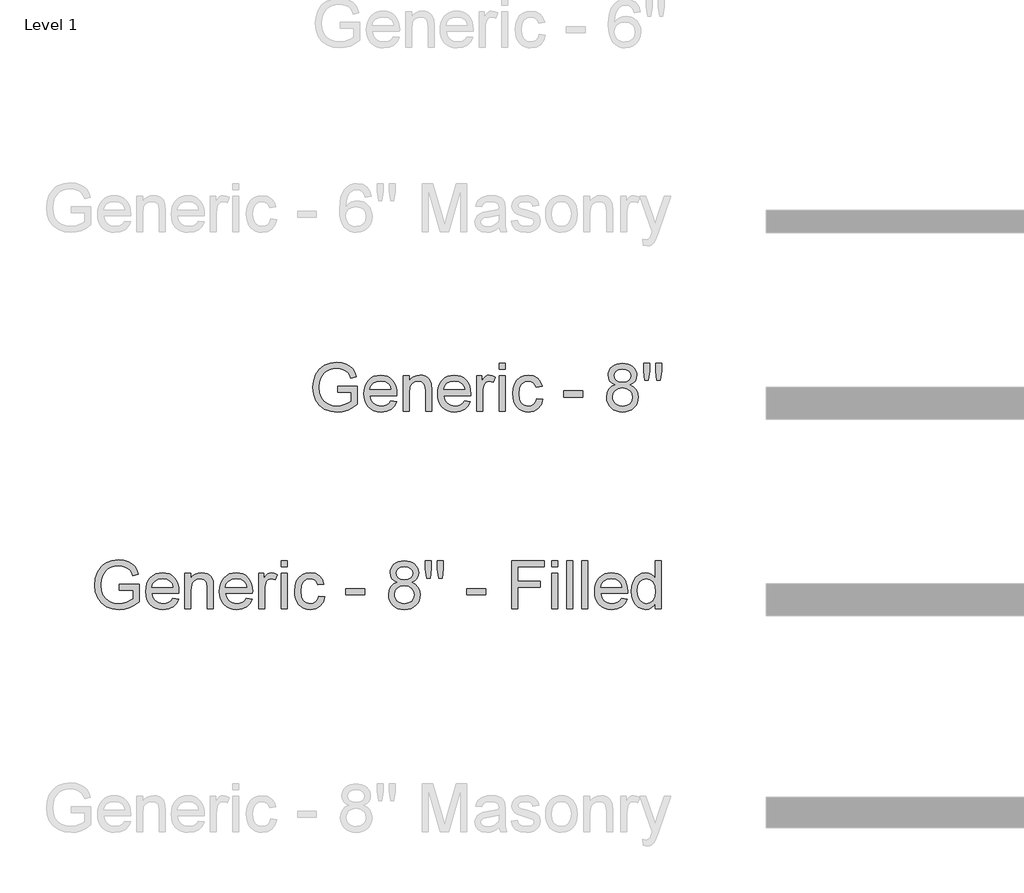
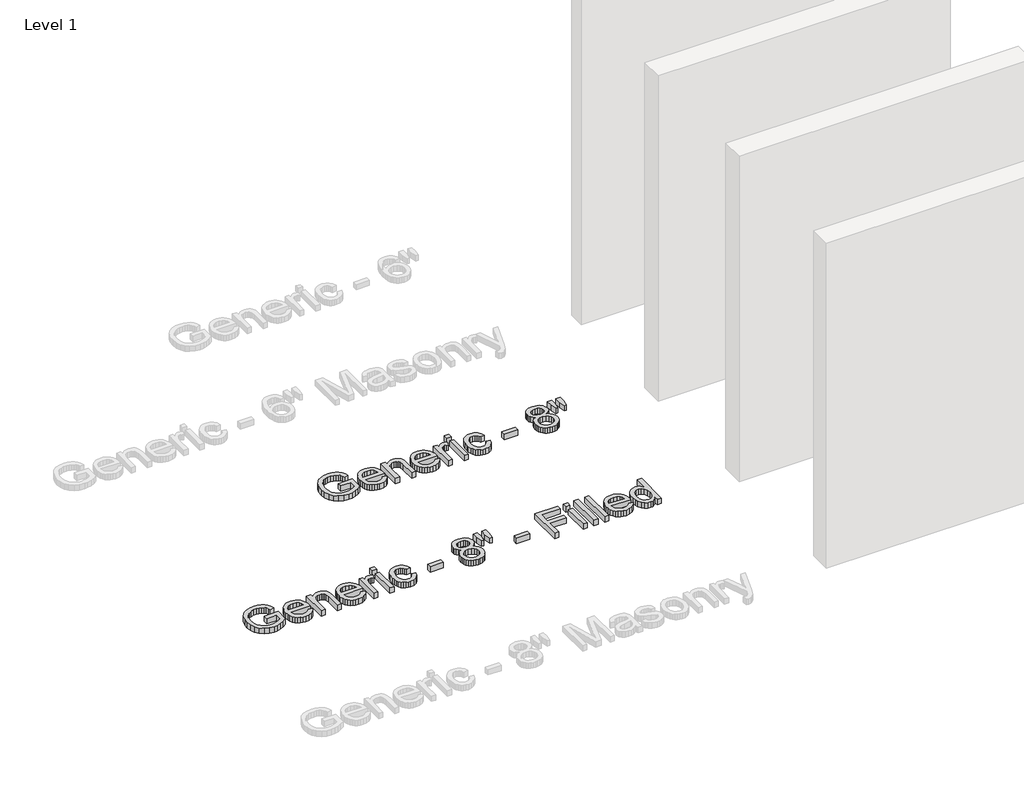
# One storey, part 23 of 42: 2 proxies.
"""IFC4 building model written with IfcOpenShell, lengths in millimetres."""

import ifcopenshell
import ifcopenshell.guid

model = None  # the IFC model being written
_history = None  # IfcOwnerHistory: only IFC2X3 demands one
_inside = {}  # id of a spatial element -> (the spatial element, [elements in it])
_under = {}  # id of a project, library or spatial element -> (it, [spatial elements below it])
_declared = {}  # id of a project -> (the project, [libraries it declares])
_typed = {}  # id of a type object -> (the type object, [elements of that type])
_made_of = {}  # id of a material, layer set ... -> (it, [elements and type objects made of it])


def new_model(schema):
    """Start an empty IFC model of exactly this schema.

    Asked for "IFC4X3", IfcOpenShell would pick the latest addendum, in which some entities
    have other attributes; the version numbers below select the first issue.
    IFC2X3 requires an IfcOwnerHistory on every rooted entity: one is made here for all.
    """
    global model, _history
    if schema == "IFC4X3":
        model = ifcopenshell.file(schema_version=(4, 3, 0, 0))
    else:
        model = ifcopenshell.file(schema=schema)
    _inside.clear()
    _under.clear()
    _declared.clear()
    _typed.clear()
    _made_of.clear()
    _history = None
    if model.schema == "IFC2X3":
        org = make("IfcOrganization", Name="unknown")
        user = make(
            "IfcPersonAndOrganization",
            ThePerson=make("IfcPerson", FamilyName="unknown"),
            TheOrganization=org,
        )
        app = make(
            "IfcApplication",
            ApplicationDeveloper=org,
            Version="unknown",
            ApplicationFullName="unknown",
            ApplicationIdentifier="unknown",
        )
        _history = make(
            "IfcOwnerHistory",
            OwningUser=user,
            OwningApplication=app,
            ChangeAction="ADDED",
            CreationDate=0,
        )
    return model


def make(cls, **values):
    """One entity of the class cls with the attributes given. An attribute that is None is left unset."""
    return model.create_entity(
        cls, **{name: value for name, value in values.items() if value is not None}
    )


def rooted(cls, **values):
    """An entity with a GlobalId (a new one), such as an element, a storey or a relation."""
    return make(cls, GlobalId=ifcopenshell.guid.new(), OwnerHistory=_history, **values)


def si_unit(unit_type, name, prefix=None):
    """IfcSIUnit, for example si_unit("LENGTHUNIT", "METRE", prefix="MILLI")."""
    return make("IfcSIUnit", UnitType=unit_type, Prefix=prefix, Name=name)


def assignment(units):
    """IfcUnitAssignment: the units of a project."""
    return None if units is None else make("IfcUnitAssignment", Units=units)


def point(xyz):
    """IfcCartesianPoint."""
    return None if xyz is None else make("IfcCartesianPoint", Coordinates=xyz)


def direction(xyz):
    """IfcDirection."""
    return None if xyz is None else make("IfcDirection", DirectionRatios=xyz)


def frame(location, z_axis=None, x_axis=None):
    """IfcAxis2Placement3D, a coordinate frame: its origin and axes. An axis left out is left unset."""
    return make(
        "IfcAxis2Placement3D",
        Location=point(location),
        Axis=direction(z_axis),
        RefDirection=direction(x_axis),
    )


def origin():
    """The frame at (0, 0, 0) with its axes left unset."""
    return frame((0.0, 0.0, 0.0))


def origin_with_axes():
    """The frame at (0, 0, 0) with the z axis (0, 0, 1) and the x axis (1, 0, 0) written out."""
    return frame((0.0, 0.0, 0.0), z_axis=(0.0, 0.0, 1.0), x_axis=(1.0, 0.0, 0.0))


def place(relative_to, where):
    """IfcLocalPlacement: puts the frame where relative to a parent placement (None: the world)."""
    return make(
        "IfcLocalPlacement", PlacementRelTo=relative_to, RelativePlacement=where
    )


def context(
    kind, dimensions, precision=None, world=None, true_north=None, identifier=None
):
    """IfcGeometricRepresentationContext, for example the 3D "Model" context."""
    return make(
        "IfcGeometricRepresentationContext",
        ContextIdentifier=identifier,
        ContextType=kind,
        CoordinateSpaceDimension=dimensions,
        Precision=precision,
        WorldCoordinateSystem=world,
        TrueNorth=true_north,
    )


def project(units=None, contexts=None):
    """IfcProject with its units and contexts."""
    return rooted(
        "IfcProject",
        Name="project",
        RepresentationContexts=contexts,
        UnitsInContext=assignment(units),
    )


def spatial(cls, under=None, at=None, **own):
    """A site, building, storey or space (cls), placed at a placement, below another one or the project."""
    s = rooted(cls, ObjectPlacement=at, **own)
    if under is not None:
        _under.setdefault(under.id(), (under, []))[1].append(s)
    return s


def polyline(points):
    """IfcPolyline through the points."""
    return make("IfcPolyline", Points=[point(p) for p in points])


def outline(outer, holes=None, kind="AREA"):
    """IfcArbitraryClosedProfileDef: a profile drawn as a closed curve; with holes, ...WithVoids."""
    if holes is None:
        return make("IfcArbitraryClosedProfileDef", ProfileType=kind, OuterCurve=outer)
    return make(
        "IfcArbitraryProfileDefWithVoids",
        ProfileType=kind,
        OuterCurve=outer,
        InnerCurves=holes,
    )


def extrude(swept, where, along, depth):
    """IfcExtrudedAreaSolid: the profile swept, set in the frame where, extruded along a direction by depth."""
    return make(
        "IfcExtrudedAreaSolid",
        SweptArea=swept,
        Position=where,
        ExtrudedDirection=direction(along),
        Depth=depth,
    )


def shape(context_of_items, identifier, shape_type, items):
    """IfcShapeRepresentation: the items that make up one representation, for example the "Body"."""
    return make(
        "IfcShapeRepresentation",
        ContextOfItems=context_of_items,
        RepresentationIdentifier=identifier,
        RepresentationType=shape_type,
        Items=items,
    )


def made_of(thing, what):
    """Note that an element or type object is made of a material, layer set ...; save() writes the relation."""
    if what is not None:
        _made_of.setdefault(what.id(), (what, []))[1].append(thing)
    return thing


def element(
    cls,
    number,
    at=None,
    inside=None,
    cuts=None,
    type_object=None,
    material=None,
    context=None,
    identifier="Body",
    shape_type=None,
    held_by="IfcProductDefinitionShape",
    body=None,
    shapes=None,
    **own,
):
    """One element of the class cls, such as IfcWall. Its Tag is "e" and its number.

    at: its placement. inside: the storey or other place that contains it. cuts: it is an
    opening in that element (IfcRelVoidsElement). A single representation is given by context,
    identifier, shape_type and body (its items); several are given by shapes. held_by: the class
    of the entity that holds the representations. save() writes the other relations.
    """
    e = rooted(cls, Tag="e%d" % number, ObjectPlacement=at, **own)
    if body is not None:
        shapes = [shape(context, identifier, shape_type, body)]
    if shapes is not None:
        e.Representation = make(held_by, Representations=shapes)
    if inside is not None:
        _inside.setdefault(inside.id(), (inside, []))[1].append(e)
    if cuts is not None:
        rooted(
            "IfcRelVoidsElement", RelatingBuildingElement=cuts, RelatedOpeningElement=e
        )
    if type_object is not None:
        _typed.setdefault(type_object.id(), (type_object, []))[1].append(e)
    return made_of(e, material)


def aggregate(whole, parts):
    """IfcRelAggregates: a whole, such as a stair, and the parts it consists of."""
    return rooted("IfcRelAggregates", RelatingObject=whole, RelatedObjects=parts)


def save(model, path):
    """Write the relations noted so far, then the file.

    IfcRelAggregates (storeys below a building ...), IfcRelContainedInSpatialStructure (elements
    in a storey), IfcRelDefinesByType, IfcRelAssociatesMaterial and IfcRelDeclares: one each for
    every whole, place, type object, material and project.
    """
    for whole, parts in _under.values():
        aggregate(whole, parts)
    for where, things in _inside.values():
        rooted(
            "IfcRelContainedInSpatialStructure",
            RelatedElements=things,
            RelatingStructure=where,
        )
    for kind, things in _typed.values():
        rooted("IfcRelDefinesByType", RelatedObjects=things, RelatingType=kind)
    for what, things in _made_of.values():
        rooted("IfcRelAssociatesMaterial", RelatedObjects=things, RelatingMaterial=what)
    for by, libraries in _declared.values():
        rooted("IfcRelDeclares", RelatingContext=by, RelatedDefinitions=libraries)
    model.write(path)


model = new_model("IFC4")

# Units and contexts
model_context = context("Model", 3, world=origin())
ifc_project = project(units=[si_unit("LENGTHUNIT", "METRE", prefix="MILLI")], contexts=[model_context])

# Site, building, storey
site = spatial("IfcSite", under=ifc_project)
building = spatial("IfcBuilding", under=site)
storey = spatial("IfcBuildingStorey", under=building, Name="Level 1", Elevation=0.0)

# Proxies
placement = place(None, origin())
element("IfcBuildingElementProxy", 1, Name="8\" Arial", ObjectType="8\" Arial", at=placement, inside=storey, context=model_context, shape_type="SweptSolid", body=[
    extrude(outline(polyline([(-15234.2304612, 12301.3438575), (-15234.2304612, 12339.4147443), (-15110.5000792, 12339.4147443), (-15110.5000792, 12225.57387), (-15140.5682722, 12204.6609073), (-15171.5845196, 12189.6593421), (-15203.474464, 12180.6249422), (-15236.1637484, 12177.6134755), (-15278.8726656, 12182.4002203), (-15317.4733474, 12196.7604547), (-15349.5398902, 12220.1922676), (-15372.6463903, 12252.1937479), (-15386.6162494, 12290.5806527), (-15391.2728691, 12333.1687394), (-15386.6348387, 12376.0635496), (-15372.7207475, 12415.9654824), (-15350.1068638, 12449.4355174), (-15335.7536004, 12462.4689404), (-15319.369456, 12473.0346339), (-15281.9306054, 12487.032377), (-15239.2123936, 12491.6982913), (-15207.8522442, 12488.9935481), (-15179.6522759, 12480.8793186), (-15155.9044449, 12467.9411657), (-15137.9007077, 12450.7646523), (-15124.5814741, 12428.5225547), (-15114.8871541, 12400.3876488), (-15149.9837528, 12390.4981412), (-15157.8191428, 12410.5652907), (-15167.3461592, 12425.7062757), (-15179.9497047, 12437.120106), (-15197.0146822, 12446.0057915), (-15217.3606713, 12451.7220013), (-15239.8072512, 12453.6274045), (-15266.083227, 12451.5732869), (-15288.5483963, 12445.4109339), (-15307.1191072, 12435.9118015), (-15321.7117078, 12423.8473457), (-15341.3048302, 12394.51343), (-15350.2276943, 12365.7743719), (-15353.2019823, 12334.7302406), (-15349.623542, 12298.3230962), (-15338.8882212, 12268.366439), (-15321.3213325, 12245.0740459), (-15297.2481888, 12228.6596938), (-15269.0761044, 12218.9281952), (-15239.2123936, 12215.6843623), (-15212.8434713, 12218.1288553), (-15187.1251745, 12225.4623342), (-15164.7901304, 12235.5656188), (-15148.570966, 12246.319529), (-15148.570966, 12301.3438575), (-15234.2304612, 12301.3438575)])), origin_with_axes(), (0.0, 0.0, 1.0), 50.8),
    extrude(outline(polyline([(-14896.7974844, 12248.9963882), (-14859.4701697, 12244.2375274), (-14872.9195283, 12216.1119162), (-14894.3808754, 12195.0874177), (-14923.370889, 12181.9819611), (-14959.4062474, 12177.6134755), (-14983.0286006, 12179.4979659), (-15004.0763357, 12185.1514368), (-15022.5494528, 12194.5738883), (-15038.4479517, 12207.7653204), (-15051.2327429, 12224.3585945), (-15060.3647366, 12243.9865718), (-15065.8439329, 12266.6492524), (-15067.6703316, 12292.3466362), (-15065.8253436, 12318.9153935), (-15060.2903794, 12342.3332644), (-15051.0654392, 12362.6002489), (-15038.1505229, 12379.7163471), (-15022.2938499, 12393.3144201), (-15004.2436394, 12403.0273295), (-14983.9998915, 12408.8550751), (-14961.5626062, 12410.7976569), (-14939.8479799, 12408.8597224), (-14920.210708, 12403.0459188), (-14902.6507903, 12393.3562461), (-14887.1682269, 12379.7907043), (-14874.5298265, 12362.7117847), (-14865.5023976, 12342.4819788), (-14860.0859402, 12319.1012865), (-14858.2804544, 12292.5697078), (-14858.503526, 12282.3084141), (-15029.5994449, 12282.3084141), (-15023.0095379, 12253.811017), (-15007.7012492, 12232.8608757), (-14985.607866, 12219.9784906), (-14958.6626754, 12215.6843623), (-14938.4003382, 12217.6734174), (-14921.3353606, 12223.6405828), (-14907.4677427, 12233.9576444), (-14896.7974844, 12248.9963882)]), holes=[polyline([(-15029.5994449, 12320.3793009), (-14896.3513412, 12320.3793009), (-14901.5005773, 12340.4929237), (-14911.5945673, 12354.881042), (-14933.7901918, 12368.2653381), (-14961.7113206, 12372.7267702), (-14987.3738495, 12369.1669192), (-15008.5935357, 12358.4873663), (-15023.3441453, 12341.8406479), (-15029.5994449, 12320.3793009)])]), origin_with_axes(), (0.0, 0.0, 1.0), 50.8),
    extrude(outline(polyline([(-14820.2095677, 12182.3723364), (-14820.2095677, 12406.0387961), (-14782.1386809, 12406.0387961), (-14782.1386809, 12374.8087718), (-14768.9123938, 12390.5539091), (-14753.0278368, 12401.8004357), (-14734.4850099, 12408.5483516), (-14713.2839131, 12410.7976569), (-14694.5180145, 12408.9852002), (-14677.3322065, 12403.5478299), (-14662.9998561, 12395.1640555), (-14652.7943303, 12384.5123865), (-14641.3805, 12356.5169004), (-14639.3728556, 12319.7100861), (-14639.3728556, 12182.3723364), (-14677.4437423, 12182.3723364), (-14677.4437423, 12314.5794392), (-14681.8308172, 12348.2632512), (-14687.9002237, 12358.2921786), (-14697.3342935, 12366.0718007), (-14709.4266333, 12371.0630278), (-14723.4708496, 12372.7267702), (-14745.7687151, 12368.9903209), (-14764.7762746, 12357.7809728), (-14772.3723273, 12348.6303898), (-14777.7980793, 12336.1244381), (-14782.1386809, 12301.0464287), (-14782.1386809, 12182.3723364), (-14820.2095677, 12182.3723364)])), origin_with_axes(), (0.0, 0.0, 1.0), 50.8),
    extrude(outline(polyline([(-14430.4291216, 12248.9963882), (-14393.1018069, 12244.2375274), (-14406.5511655, 12216.1119162), (-14428.0125126, 12195.0874177), (-14457.0025262, 12181.9819611), (-14493.0378846, 12177.6134755), (-14516.6602378, 12179.4979659), (-14537.7079729, 12185.1514368), (-14556.18109, 12194.5738883), (-14572.0795889, 12207.7653204), (-14584.8643801, 12224.3585945), (-14593.9963739, 12243.9865718), (-14599.4755701, 12266.6492524), (-14601.3019688, 12292.3466362), (-14599.4569808, 12318.9153935), (-14593.9220167, 12342.3332644), (-14584.6970764, 12362.6002489), (-14571.7821601, 12379.7163471), (-14555.9254871, 12393.3144201), (-14537.8752766, 12403.0273295), (-14517.6315287, 12408.8550751), (-14495.1942434, 12410.7976569), (-14473.4796172, 12408.8597224), (-14453.8423452, 12403.0459188), (-14436.2824275, 12393.3562461), (-14420.7998641, 12379.7907043), (-14408.1614637, 12362.7117847), (-14399.1340348, 12342.4819788), (-14393.7175774, 12319.1012865), (-14391.9120916, 12292.5697078), (-14392.1351632, 12282.3084141), (-14563.2310821, 12282.3084141), (-14556.6411751, 12253.811017), (-14541.3328865, 12232.8608757), (-14519.2395032, 12219.9784906), (-14492.2943126, 12215.6843623), (-14472.0319754, 12217.6734174), (-14454.9669978, 12223.6405828), (-14441.0993799, 12233.9576444), (-14430.4291216, 12248.9963882)]), holes=[polyline([(-14563.2310821, 12320.3793009), (-14429.9829784, 12320.3793009), (-14435.1322146, 12340.4929237), (-14445.2262045, 12354.881042), (-14467.421829, 12368.2653381), (-14495.3429578, 12372.7267702), (-14521.0054867, 12369.1669192), (-14542.2251729, 12358.4873663), (-14556.9757826, 12341.8406479), (-14563.2310821, 12320.3793009)])]), origin_with_axes(), (0.0, 0.0, 1.0), 50.8),
    extrude(outline(polyline([(-14353.8412049, 12182.3723364), (-14353.8412049, 12406.0387961), (-14320.529179, 12406.0387961), (-14320.529179, 12372.9498418), (-14308.2230623, 12392.1339996), (-14296.8835892, 12403.4362941), (-14285.5069374, 12408.9573162), (-14273.0892849, 12410.7976569), (-14254.1281988, 12407.8605475), (-14234.8696838, 12399.0492192), (-14247.5847651, 12364.9192641), (-14260.9690612, 12370.7748937), (-14274.3533573, 12372.7267702), (-14285.7207144, 12370.8492509), (-14295.8797669, 12365.2166929), (-14304.086943, 12356.2566502), (-14309.5986705, 12344.3966767), (-14314.2274062, 12323.1305173), (-14315.7703181, 12299.9310707), (-14315.7703181, 12182.3723364), (-14353.8412049, 12182.3723364)])), origin_with_axes(), (0.0, 0.0, 1.0), 50.8),
    extrude(outline(polyline([(-14211.0753795, 12448.8685437), (-14211.0753795, 12486.9394305), (-14173.0044928, 12486.9394305), (-14173.0044928, 12448.8685437), (-14211.0753795, 12448.8685437)])), origin_with_axes(), (0.0, 0.0, 1.0), 50.8),
    extrude(outline(polyline([(-14211.0753795, 12182.3723364), (-14211.0753795, 12406.0387961), (-14173.0044928, 12406.0387961), (-14173.0044928, 12182.3723364), (-14211.0753795, 12182.3723364)])), origin_with_axes(), (0.0, 0.0, 1.0), 50.8),
    extrude(outline(polyline([(-13973.1323373, 12263.2729708), (-13935.0614505, 12258.5141099), (-13945.6759409, 12224.6536996), (-13965.62226, 12199.065528), (-13993.0228885, 12182.9764886), (-14026.000307, 12177.6134755), (-14047.3524419, 12179.4840239), (-14066.4970974, 12185.0956689), (-14083.4342736, 12194.4484105), (-14098.1639703, 12207.5422488), (-14110.0866827, 12224.1308756), (-14118.6029058, 12243.9679825), (-14123.7126397, 12267.0535697), (-14125.4158843, 12293.387637), (-14122.5066589, 12327.2666366), (-14113.7789824, 12356.6284362), (-14099.0934353, 12380.3390886), (-14078.3105977, 12397.2646464), (-14053.4474087, 12407.4144043), (-14026.5208074, 12410.7976569), (-13994.3520235, 12406.1503319), (-13968.6337267, 12392.2083568), (-13950.1838462, 12369.7153036), (-13939.8203114, 12339.4147443), (-13977.8911981, 12334.6558834), (-13984.7971232, 12351.2654231), (-13995.5510333, 12363.1718699), (-14009.558071, 12370.3380451), (-14026.2233786, 12372.7267702), (-14050.8263174, 12368.0236772), (-14070.3543772, 12353.9143984), (-14083.0973425, 12329.6367724), (-14087.3449976, 12294.4286378), (-14083.190289, 12258.7464762), (-14070.7261632, 12234.3851983), (-14051.5513001, 12220.3595713), (-14027.2643794, 12215.6843623), (-14007.5504266, 12218.6028824), (-13991.3870301, 12227.3584428), (-13979.6292977, 12242.1741151), (-13973.1323373, 12263.2729708)])), origin_with_axes(), (0.0, 0.0, 1.0), 50.8),
    extrude(outline(polyline([(-13801.8133469, 12272.7906924), (-13801.8133469, 12310.8615792), (-13682.8418258, 12310.8615792), (-13682.8418258, 12272.7906924), (-13801.8133469, 12272.7906924)])), origin_with_axes(), (0.0, 0.0, 1.0), 50.8),
    extrude(outline(polyline([(-13475.087807, 12350.1221812), (-13495.4709747, 12360.1604033), (-13509.7754411, 12373.767771), (-13518.2242781, 12390.6654449), (-13521.040557, 12410.5745853), (-13519.5069398, 12426.1012983), (-13514.906088, 12440.3360549), (-13507.2380017, 12453.2788552), (-13496.5026808, 12464.9296991), (-13483.2159785, 12474.5589565), (-13467.8937478, 12481.4369976), (-13431.1427014, 12486.9394305), (-13394.1685834, 12481.3068725), (-13378.679049, 12474.2661751), (-13365.1878644, 12464.4091986), (-13354.2573559, 12452.5306358), (-13346.4498498, 12439.4251792), (-13341.7653462, 12425.0928288), (-13340.2038449, 12409.5335845), (-13342.9829453, 12390.2657749), (-13351.3202464, 12373.6562352), (-13365.3086948, 12360.1325193), (-13385.041237, 12350.1221812), (-13361.6094241, 12338.0484307), (-13344.5537412, 12320.2677651), (-13334.1530277, 12297.6352921), (-13330.6861233, 12271.0061196), (-13332.4056335, 12252.0171495), (-13337.5641643, 12234.6082699), (-13346.1617156, 12218.7794808), (-13358.1982875, 12204.5307822), (-13373.0418437, 12192.7544605), (-13390.060348, 12184.3428022), (-13409.2538004, 12179.2958072), (-13430.622201, 12177.6134755), (-13451.9906015, 12179.3027782), (-13471.184054, 12184.3706862), (-13488.2025583, 12192.8171994), (-13503.0461145, 12204.642318), (-13515.0826863, 12218.9909341), (-13523.6802377, 12235.0079398), (-13528.8387685, 12252.6933353), (-13530.5582787, 12272.0471204), (-13526.9519545, 12299.7079991), (-13516.1329818, 12322.4613025), (-13498.6590396, 12339.5262801), (-13475.087807, 12350.1221812)]), holes=[polyline([(-13482.9696703, 12409.4592273), (-13479.5957123, 12392.840393), (-13469.4738384, 12379.5676327), (-13452.9014773, 12370.8678402), (-13430.1760578, 12367.9679093), (-13407.9804334, 12370.8492509), (-13391.6590278, 12379.4932755), (-13381.6208057, 12392.3198926), (-13378.2747317, 12407.7490117), (-13381.7323415, 12423.7636938), (-13392.105171, 12437.0085702), (-13408.6496482, 12445.9035503), (-13430.622201, 12448.8685437), (-13452.7341736, 12445.9686129), (-13469.2507668, 12437.2688204), (-13479.5399444, 12424.5165605), (-13482.9696703, 12409.4592273)]), polyline([(-13492.487392, 12273.3855501), (-13490.8980068, 12258.8208334), (-13486.1298513, 12244.7208492), (-13477.3278177, 12232.4240271), (-13463.6367981, 12223.2687968), (-13447.2410354, 12217.5804709), (-13430.3247722, 12215.6843623), (-13404.4112877, 12219.6717672), (-13384.9668798, 12231.6339819), (-13372.8094775, 12249.7492549), (-13368.75701, 12272.1958348), (-13372.9396026, 12295.0234955), (-13385.4873802, 12313.5384384), (-13405.3779314, 12325.8073765), (-13431.5888446, 12329.8970226), (-13457.1398377, 12325.8631444), (-13476.389058, 12313.76151), (-13488.4628085, 12295.5997638), (-13492.487392, 12273.3855501)])]), origin_with_axes(), (0.0, 0.0, 1.0), 50.8),
    extrude(outline(polyline([(-13288.0794473, 12377.485631), (-13297.3740973, 12436.3021768), (-13297.3740973, 12486.9394305), (-13259.3032106, 12486.9394305), (-13259.3032106, 12436.3021768), (-13267.6312171, 12377.485631), (-13288.0794473, 12377.485631)])), origin_with_axes(), (0.0, 0.0, 1.0), 50.8),
    extrude(outline(polyline([(-13212.1607453, 12377.485631), (-13221.2323238, 12436.3021768), (-13221.2323238, 12486.9394305), (-13183.1614371, 12486.9394305), (-13183.1614371, 12436.3021768), (-13192.0843011, 12377.485631), (-13212.1607453, 12377.485631)])), origin_with_axes(), (0.0, 0.0, 1.0), 50.8),
])
element("IfcBuildingElementProxy", 2, Name="8\" Arial", ObjectType="8\" Arial", at=placement, inside=storey, context=model_context, shape_type="SweptSolid", body=[
    extrude(outline(polyline([(-16615.2716605, 11050.690593), (-16615.2716605, 11088.7614797), (-16491.5412786, 11088.7614797), (-16491.5412786, 10974.9206055), (-16521.6094716, 10954.0076428), (-16552.6257189, 10939.0060775), (-16584.5156634, 10929.9716776), (-16617.2049477, 10926.960211), (-16659.9138649, 10931.7469558), (-16698.5145467, 10946.1071902), (-16730.5810895, 10969.5390031), (-16753.6875896, 11001.5404833), (-16767.6574487, 11039.9273882), (-16772.3140684, 11082.5154749), (-16767.676038, 11125.410285), (-16753.7619468, 11165.3122179), (-16731.1480632, 11198.7822528), (-16716.7947998, 11211.8156759), (-16700.4106553, 11222.3813694), (-16662.9718048, 11236.3791124), (-16620.253593, 11241.0450268), (-16588.8934436, 11238.3402836), (-16560.6934752, 11230.2260541), (-16536.9456442, 11217.2879011), (-16518.941907, 11200.1113878), (-16505.6226734, 11177.8692901), (-16495.9283534, 11149.7343843), (-16531.0249521, 11139.8448766), (-16538.8603421, 11159.9120262), (-16548.3873585, 11175.0530111), (-16560.990904, 11186.4668415), (-16578.0558816, 11195.3525269), (-16598.4018706, 11201.0687367), (-16620.8484506, 11202.97414), (-16647.1244264, 11200.9200223), (-16669.5895956, 11194.7576693), (-16688.1603065, 11185.2585369), (-16702.7529071, 11173.1940811), (-16722.3460295, 11143.8601655), (-16731.2688936, 11115.1211074), (-16734.2431816, 11084.0769761), (-16730.6647414, 11047.6698317), (-16719.9294205, 11017.7131745), (-16702.3625318, 10994.4207813), (-16678.2893881, 10978.0064293), (-16650.1173037, 10968.2749307), (-16620.253593, 10965.0310978), (-16593.8846707, 10967.4755907), (-16568.1663739, 10974.8090697), (-16545.8313297, 10984.9123543), (-16529.6121653, 10995.6662645), (-16529.6121653, 11050.690593), (-16615.2716605, 11050.690593)])), origin_with_axes(), (0.0, 0.0, 1.0), 50.8),
    extrude(outline(polyline([(-16277.8386837, 10998.3431237), (-16240.511369, 10993.5842628), (-16253.9607277, 10965.4586517), (-16275.4220747, 10944.4341532), (-16304.4120883, 10931.3286966), (-16340.4474467, 10926.960211), (-16364.0697999, 10928.8447013), (-16385.117535, 10934.4981722), (-16403.5906521, 10943.9206238), (-16419.4891511, 10957.1120559), (-16432.2739423, 10973.70533), (-16441.405936, 10993.3333073), (-16446.8851322, 11015.9959879), (-16448.7115309, 11041.6933717), (-16446.8665429, 11068.262129), (-16441.3315788, 11091.6799999), (-16432.1066386, 11111.9469844), (-16419.1917223, 11129.0630825), (-16403.3350492, 11142.6611556), (-16385.2848387, 11152.3740649), (-16365.0410909, 11158.2018105), (-16342.6038055, 11160.1443924), (-16320.8891793, 11158.2064579), (-16301.2519073, 11152.3926542), (-16283.6919896, 11142.7029815), (-16268.2094262, 11129.1374397), (-16255.5710258, 11112.0585202), (-16246.5435969, 11091.8287143), (-16241.1271396, 11068.448022), (-16239.3216538, 11041.9164433), (-16239.5447254, 11031.6551496), (-16410.6406442, 11031.6551496), (-16404.0507373, 11003.1577524), (-16388.7424486, 10982.2076111), (-16366.6490653, 10969.3252261), (-16339.7038747, 10965.0310978), (-16319.4415375, 10967.0201529), (-16302.37656, 10972.9873182), (-16288.508942, 10983.3043798), (-16277.8386837, 10998.3431237)]), holes=[polyline([(-16410.6406442, 11069.7260364), (-16277.3925405, 11069.7260364), (-16282.5417767, 11089.8396591), (-16292.6357667, 11104.2277775), (-16314.8313911, 11117.6120736), (-16342.7525199, 11122.0735057), (-16368.4150488, 11118.5136547), (-16389.634735, 11107.8341017), (-16404.3853447, 11091.1873834), (-16410.6406442, 11069.7260364)])]), origin_with_axes(), (0.0, 0.0, 1.0), 50.8),
    extrude(outline(polyline([(-16201.250767, 10931.7190719), (-16201.250767, 11155.3855316), (-16163.1798803, 11155.3855316), (-16163.1798803, 11124.1555073), (-16149.9535932, 11139.9006445), (-16134.0690362, 11151.1471711), (-16115.5262093, 11157.8950871), (-16094.3251124, 11160.1443924), (-16075.5592139, 11158.3319356), (-16058.3734059, 11152.8945653), (-16044.0410554, 11144.510791), (-16033.8355296, 11133.859122), (-16022.4216993, 11105.8636359), (-16020.4140549, 11069.0568216), (-16020.4140549, 10931.7190719), (-16058.4849417, 10931.7190719), (-16058.4849417, 11063.9261747), (-16062.8720165, 11097.6099866), (-16068.941423, 11107.6389141), (-16078.3754929, 11115.4185362), (-16090.4678326, 11120.4097633), (-16104.5120489, 11122.0735057), (-16126.8099145, 11118.3370563), (-16145.8174739, 11107.1277083), (-16153.4135267, 11097.9771253), (-16158.8392787, 11085.4711736), (-16163.1798803, 11050.3931642), (-16163.1798803, 10931.7190719), (-16201.250767, 10931.7190719)])), origin_with_axes(), (0.0, 0.0, 1.0), 50.8),
    extrude(outline(polyline([(-15811.4703209, 10998.3431237), (-15774.1430062, 10993.5842628), (-15787.5923649, 10965.4586517), (-15809.0537119, 10944.4341532), (-15838.0437255, 10931.3286966), (-15874.0790839, 10926.960211), (-15897.7014371, 10928.8447013), (-15918.7491723, 10934.4981722), (-15937.2222893, 10943.9206238), (-15953.1207883, 10957.1120559), (-15965.9055795, 10973.70533), (-15975.0375732, 10993.3333073), (-15980.5167694, 11015.9959879), (-15982.3431682, 11041.6933717), (-15980.4981801, 11068.262129), (-15974.963216, 11091.6799999), (-15965.7382758, 11111.9469844), (-15952.8233595, 11129.0630825), (-15936.9666864, 11142.6611556), (-15918.916476, 11152.3740649), (-15898.6727281, 11158.2018105), (-15876.2354428, 11160.1443924), (-15854.5208165, 11158.2064579), (-15834.8835445, 11152.3926542), (-15817.3236268, 11142.7029815), (-15801.8410635, 11129.1374397), (-15789.202663, 11112.0585202), (-15780.1752341, 11091.8287143), (-15774.7587768, 11068.448022), (-15772.953291, 11041.9164433), (-15773.1763626, 11031.6551496), (-15944.2722814, 11031.6551496), (-15937.6823745, 11003.1577524), (-15922.3740858, 10982.2076111), (-15900.2807025, 10969.3252261), (-15873.3355119, 10965.0310978), (-15853.0731747, 10967.0201529), (-15836.0081972, 10972.9873182), (-15822.1405792, 10983.3043798), (-15811.4703209, 10998.3431237)]), holes=[polyline([(-15944.2722814, 11069.7260364), (-15811.0241777, 11069.7260364), (-15816.1734139, 11089.8396591), (-15826.2674039, 11104.2277775), (-15848.4630283, 11117.6120736), (-15876.3841572, 11122.0735057), (-15902.046686, 11118.5136547), (-15923.2663722, 11107.8341017), (-15938.0169819, 11091.1873834), (-15944.2722814, 11069.7260364)])]), origin_with_axes(), (0.0, 0.0, 1.0), 50.8),
    extrude(outline(polyline([(-15734.8824042, 10931.7190719), (-15734.8824042, 11155.3855316), (-15701.5703783, 11155.3855316), (-15701.5703783, 11122.2965773), (-15689.2642616, 11141.480735), (-15677.9247885, 11152.7830295), (-15666.5481368, 11158.3040517), (-15654.1304843, 11160.1443924), (-15635.1693981, 11157.207283), (-15615.9108831, 11148.3959547), (-15628.6259644, 11114.2659996), (-15642.0102605, 11120.1216291), (-15655.3945567, 11122.0735057), (-15666.7619137, 11120.1959863), (-15676.9209663, 11114.5634284), (-15685.1281423, 11105.6033857), (-15690.6398698, 11093.7434122), (-15695.2686056, 11072.4772528), (-15696.8115175, 11049.2778062), (-15696.8115175, 10931.7190719), (-15734.8824042, 10931.7190719)])), origin_with_axes(), (0.0, 0.0, 1.0), 50.8),
    extrude(outline(polyline([(-15592.1165789, 11198.2152792), (-15592.1165789, 11236.2861659), (-15554.0456921, 11236.2861659), (-15554.0456921, 11198.2152792), (-15592.1165789, 11198.2152792)])), origin_with_axes(), (0.0, 0.0, 1.0), 50.8),
    extrude(outline(polyline([(-15592.1165789, 10931.7190719), (-15592.1165789, 11155.3855316), (-15554.0456921, 11155.3855316), (-15554.0456921, 10931.7190719), (-15592.1165789, 10931.7190719)])), origin_with_axes(), (0.0, 0.0, 1.0), 50.8),
    extrude(outline(polyline([(-15354.1735366, 11012.6197062), (-15316.1026499, 11007.8608454), (-15326.7171403, 10974.0004351), (-15346.6634594, 10948.4122634), (-15374.0640878, 10932.3232241), (-15407.0415063, 10926.960211), (-15428.3936413, 10928.8307593), (-15447.5382968, 10934.4424043), (-15464.4754729, 10943.795146), (-15479.2051696, 10956.8889843), (-15491.127882, 10973.477611), (-15499.6441052, 10993.314718), (-15504.753839, 11016.4003051), (-15506.4570837, 11042.7343725), (-15503.5478582, 11076.6133721), (-15494.8201818, 11105.9751717), (-15480.1346346, 11129.6858241), (-15459.351797, 11146.6113819), (-15434.488608, 11156.7611398), (-15407.5620067, 11160.1443924), (-15375.3932228, 11155.4970674), (-15349.674926, 11141.5550922), (-15331.2250456, 11119.062039), (-15320.8615107, 11088.7614797), (-15358.9323975, 11084.0026189), (-15365.8383225, 11100.6121586), (-15376.5922327, 11112.5186054), (-15390.5992703, 11119.6847806), (-15407.2645779, 11122.0735057), (-15431.8675167, 11117.3704127), (-15451.3955766, 11103.2611339), (-15464.1385418, 11078.9835078), (-15468.3861969, 11043.7753733), (-15464.2314883, 11008.0932116), (-15451.7673626, 10983.7319337), (-15432.5924994, 10969.7063068), (-15408.3055787, 10965.0310978), (-15388.5916259, 10967.9496179), (-15372.4282294, 10976.7051783), (-15360.6704971, 10991.5208505), (-15354.1735366, 11012.6197062)])), origin_with_axes(), (0.0, 0.0, 1.0), 50.8),
    extrude(outline(polyline([(-15182.8545462, 11022.1374279), (-15182.8545462, 11060.2083147), (-15063.8830251, 11060.2083147), (-15063.8830251, 11022.1374279), (-15182.8545462, 11022.1374279)])), origin_with_axes(), (0.0, 0.0, 1.0), 50.8),
    extrude(outline(polyline([(-14856.1290063, 11099.4689166), (-14876.512174, 11109.5071387), (-14890.8166405, 11123.1145065), (-14899.2654774, 11140.0121803), (-14902.0817564, 11159.9213208), (-14900.5481391, 11175.4480338), (-14895.9472873, 11189.6827904), (-14888.279201, 11202.6255906), (-14877.5438802, 11214.2764345), (-14864.2571779, 11223.905692), (-14848.9349472, 11230.7837331), (-14812.1839007, 11236.2861659), (-14775.2097827, 11230.653608), (-14759.7202483, 11223.6129105), (-14746.2290637, 11213.7559341), (-14735.2985552, 11201.8773713), (-14727.4910491, 11188.7719147), (-14722.8065455, 11174.4395642), (-14721.2450443, 11158.88032), (-14724.0241447, 11139.6125104), (-14732.3614458, 11123.0029707), (-14746.3498942, 11109.4792548), (-14766.0824363, 11099.4689166), (-14742.6506234, 11087.3951662), (-14725.5949405, 11069.6145006), (-14715.1942271, 11046.9820276), (-14711.7273226, 11020.3528551), (-14713.4468329, 11001.363885), (-14718.6053637, 10983.9550053), (-14727.202915, 10968.1262163), (-14739.2394868, 10953.8775177), (-14754.083043, 10942.101196), (-14771.1015473, 10933.6895377), (-14790.2949998, 10928.6425427), (-14811.6634003, 10926.960211), (-14833.0318009, 10928.6495137), (-14852.2252533, 10933.7174216), (-14869.2437576, 10942.1639349), (-14884.0873138, 10953.9890535), (-14896.1238857, 10968.3376695), (-14904.721437, 10984.3546753), (-14909.8799678, 11002.0400708), (-14911.5994781, 11021.3938559), (-14907.9931538, 11049.0547346), (-14897.1741811, 11071.808038), (-14879.700239, 11088.8730155), (-14856.1290063, 11099.4689166)]), holes=[polyline([(-14864.0108696, 11158.8059628), (-14860.6369116, 11142.1871284), (-14850.5150377, 11128.9143681), (-14833.9426766, 11120.2145756), (-14811.2172571, 11117.3146448), (-14789.0216327, 11120.1959863), (-14772.7002272, 11128.8400109), (-14762.6620051, 11141.666628), (-14759.315931, 11157.0957472), (-14762.7735409, 11173.1104293), (-14773.1463704, 11186.3553057), (-14789.6908475, 11195.2502858), (-14811.6634003, 11198.2152792), (-14833.7753729, 11195.3153483), (-14850.2919661, 11186.6155559), (-14860.5811437, 11173.8632959), (-14864.0108696, 11158.8059628)]), polyline([(-14873.5285913, 11022.7322855), (-14871.9392061, 11008.1675688), (-14867.1710507, 10994.0675846), (-14858.369017, 10981.7707626), (-14844.6779974, 10972.6155322), (-14828.2822347, 10966.9272064), (-14811.3659715, 10965.0310978), (-14785.4524871, 10969.0185027), (-14766.0080791, 10980.9807173), (-14753.8506768, 10999.0959903), (-14749.7982093, 11021.5425703), (-14753.9808019, 11044.3702309), (-14766.5285795, 11062.8851739), (-14786.4191307, 11075.154112), (-14812.6300439, 11079.243758), (-14838.181037, 11075.2098799), (-14857.4302574, 11063.1082455), (-14869.5040078, 11044.9464992), (-14873.5285913, 11022.7322855)])]), origin_with_axes(), (0.0, 0.0, 1.0), 50.8),
    extrude(outline(polyline([(-14669.1206466, 11126.8323665), (-14678.4152967, 11185.6489122), (-14678.4152967, 11236.2861659), (-14640.3444099, 11236.2861659), (-14640.3444099, 11185.6489122), (-14648.6724164, 11126.8323665), (-14669.1206466, 11126.8323665)])), origin_with_axes(), (0.0, 0.0, 1.0), 50.8),
    extrude(outline(polyline([(-14593.2019447, 11126.8323665), (-14602.2735232, 11185.6489122), (-14602.2735232, 11236.2861659), (-14564.2026364, 11236.2861659), (-14564.2026364, 11185.6489122), (-14573.1255005, 11126.8323665), (-14593.2019447, 11126.8323665)])), origin_with_axes(), (0.0, 0.0, 1.0), 50.8),
    extrude(outline(polyline([(-14416.6779502, 11022.1374279), (-14416.6779502, 11060.2083147), (-14297.7064291, 11060.2083147), (-14297.7064291, 11022.1374279), (-14416.6779502, 11022.1374279)])), origin_with_axes(), (0.0, 0.0, 1.0), 50.8),
    extrude(outline(polyline([(-14131.1462995, 10931.7190719), (-14131.1462995, 11236.2861659), (-13926.5152832, 11236.2861659), (-13926.5152832, 11198.2152792), (-14093.0754128, 11198.2152792), (-14093.0754128, 11107.7969231), (-13950.3095874, 11107.7969231), (-13950.3095874, 11069.7260364), (-14093.0754128, 11069.7260364), (-14093.0754128, 10931.7190719), (-14131.1462995, 10931.7190719)])), origin_with_axes(), (0.0, 0.0, 1.0), 50.8),
    extrude(outline(polyline([(-13878.9266747, 11198.2152792), (-13878.9266747, 11236.2861659), (-13840.855788, 11236.2861659), (-13840.855788, 11198.2152792), (-13878.9266747, 11198.2152792)])), origin_with_axes(), (0.0, 0.0, 1.0), 50.8),
    extrude(outline(polyline([(-13878.9266747, 10931.7190719), (-13878.9266747, 11155.3855316), (-13840.855788, 11155.3855316), (-13840.855788, 10931.7190719), (-13878.9266747, 10931.7190719)])), origin_with_axes(), (0.0, 0.0, 1.0), 50.8),
    extrude(outline(polyline([(-13783.7494578, 10931.7190719), (-13783.7494578, 11236.2861659), (-13745.6785711, 11236.2861659), (-13745.6785711, 10931.7190719), (-13783.7494578, 10931.7190719)])), origin_with_axes(), (0.0, 0.0, 1.0), 50.8),
    extrude(outline(polyline([(-13688.572241, 10931.7190719), (-13688.572241, 11236.2861659), (-13650.5013542, 11236.2861659), (-13650.5013542, 10931.7190719), (-13688.572241, 10931.7190719)])), origin_with_axes(), (0.0, 0.0, 1.0), 50.8),
    extrude(outline(polyline([(-13436.7987594, 10998.3431237), (-13399.4714446, 10993.5842628), (-13412.9208033, 10965.4586517), (-13434.3821504, 10944.4341532), (-13463.372164, 10931.3286966), (-13499.4075224, 10926.960211), (-13523.0298756, 10928.8447013), (-13544.0776107, 10934.4981722), (-13562.5507277, 10943.9206238), (-13578.4492267, 10957.1120559), (-13591.2340179, 10973.70533), (-13600.3660116, 10993.3333073), (-13605.8452078, 11015.9959879), (-13607.6716066, 11041.6933717), (-13605.8266185, 11068.262129), (-13600.2916544, 11091.6799999), (-13591.0667142, 11111.9469844), (-13578.1517979, 11129.0630825), (-13562.2951249, 11142.6611556), (-13544.2449144, 11152.3740649), (-13524.0011665, 11158.2018105), (-13501.5638812, 11160.1443924), (-13479.8492549, 11158.2064579), (-13460.211983, 11152.3926542), (-13442.6520653, 11142.7029815), (-13427.1695019, 11129.1374397), (-13414.5311014, 11112.0585202), (-13405.5036725, 11091.8287143), (-13400.0872152, 11068.448022), (-13398.2817294, 11041.9164433), (-13398.504801, 11031.6551496), (-13569.6007198, 11031.6551496), (-13563.0108129, 11003.1577524), (-13547.7025242, 10982.2076111), (-13525.609141, 10969.3252261), (-13498.6639504, 10965.0310978), (-13478.4016132, 10967.0201529), (-13461.3366356, 10972.9873182), (-13447.4690177, 10983.3043798), (-13436.7987594, 10998.3431237)]), holes=[polyline([(-13569.6007198, 11069.7260364), (-13436.3526162, 11069.7260364), (-13441.5018523, 11089.8396591), (-13451.5958423, 11104.2277775), (-13473.7914667, 11117.6120736), (-13501.7125956, 11122.0735057), (-13527.3751245, 11118.5136547), (-13548.5948106, 11107.8341017), (-13563.3454203, 11091.1873834), (-13569.6007198, 11069.7260364)])]), origin_with_axes(), (0.0, 0.0, 1.0), 50.8),
    extrude(outline(polyline([(-13222.2038782, 10931.7190719), (-13222.2038782, 10967.6335998), (-13233.5944718, 10949.8389922), (-13247.3923799, 10937.1285582), (-13263.5976023, 10929.5022978), (-13282.2101391, 10926.960211), (-13306.8223726, 10930.6408924), (-13329.3526044, 10941.6829368), (-13348.4252263, 10959.314888), (-13362.6646303, 10982.7652901), (-13371.5317265, 11011.086089), (-13374.4874252, 11043.3292301), (-13371.7640927, 11075.1727013), (-13363.5940953, 11103.9303487), (-13349.9867276, 11127.9663138), (-13330.9512842, 11145.6447383), (-13307.9284359, 11156.5194789), (-13282.3588535, 11160.1443924), (-13263.7323748, 11157.551185), (-13247.2622548, 11149.7715629), (-13233.3016904, 11137.8465268), (-13222.2038782, 11122.8170777), (-13222.2038782, 11236.2861659), (-13184.1329914, 11236.2861659), (-13184.1329914, 10931.7190719), (-13222.2038782, 10931.7190719)]), holes=[polyline([(-13336.4165384, 11043.4779445), (-13332.1224101, 11009.0412659), (-13319.2400251, 10984.549863), (-13300.5205998, 10969.9107891), (-13278.7153507, 10965.0310978), (-13256.9193962, 10969.6877175), (-13238.6739981, 10983.6575765), (-13226.3214081, 11007.2009252), (-13222.2038782, 11040.5780137), (-13226.3957654, 11077.0688099), (-13238.9714269, 11102.3688475), (-13257.6815575, 11117.1473411), (-13280.2768519, 11122.0735057), (-13302.3051726, 11117.3425288), (-13320.3553831, 11103.1495981), (-13332.4012496, 11078.7697309), (-13336.4165384, 11043.4779445)])]), origin_with_axes(), (0.0, 0.0, 1.0), 50.8),
])

save(model, "model.ifc")

# Revit data of these elements
# Elements 1, 2 (IfcBuildingElementProxy, "8\" Arial")
#   Phase Created = New Construction
